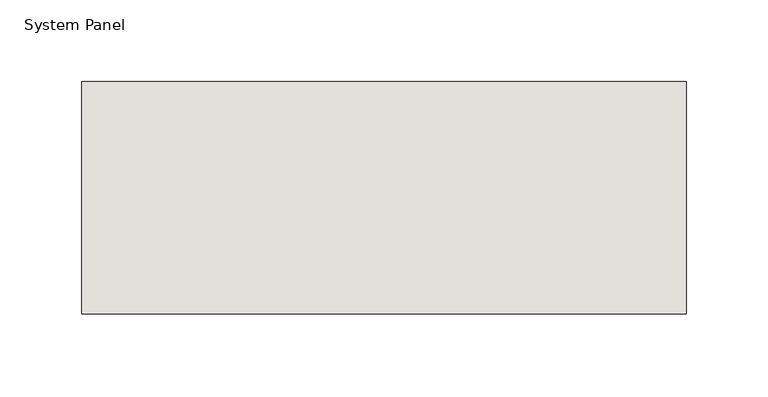
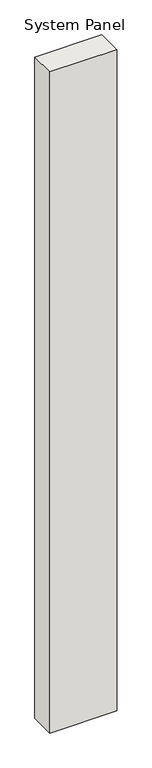
"""IFC4 building model written with IfcOpenShell, lengths in millimetres: wall geometry, System Panel : NLRS_21_CWP_hsb-vulling minerale wol 142 _gen_rsf."""

from ifc_helpers import new_model, si_unit, origin, origin_with_axes, place, context, project, spatial, polyline, outline, extrude, source, transform, mapped, element, save


def system_panel_4b5b3d98(model_context):
    return source(origin(), model_context, "Body", "SweptSolid", [
        extrude(outline(polyline([(184.5, -71.0), (-184.5, -71.0), (-184.5, 71.0), (184.5, 71.0), (184.5, -71.0)])), origin_with_axes(), (0.0, 0.0, 1.0), 3849.0),
    ])


if __name__ == "__main__":
    model = new_model("IFC4")
    model_context = context("Model", 3, world=origin())
    ifc_project = project(units=[si_unit("LENGTHUNIT", "METRE", prefix="MILLI")], contexts=[model_context])
    site = spatial("IfcSite", under=ifc_project)
    building = spatial("IfcBuilding", under=site)
    placement = place(None, origin())
    system_panel_shape = system_panel_4b5b3d98(model_context)
    element("IfcWall", 1, ObjectType="System Panel : NLRS_21_CWP_hsb-vulling minerale wol 142 _gen_rsf", at=placement, inside=building, context=model_context, shape_type="MappedRepresentation", body=[
        mapped(system_panel_shape, transform((0.0, 0.0, 0.0), x_axis=(1.0, 0.0, 0.0), y_axis=(0.0, 1.0, 0.0), z_axis=(0.0, 0.0, 1.0))),
    ])
    save(model, "model.ifc")

# Revit data of these elements
# Type "System Panel : NLRS_21_CWP_hsb-vulling minerale wol 142 _gen_rsf"
#   Type IfcGUID = "07M7mRoiH1CR8m_RSKIwpC"
#   Assembly Code = "21.23"
#   IfcExportAs = "IfcWall"
# Element 1 (IfcWall, "System Panel : NLRS_21_CWP_hsb-vulling minerale wol 142 _gen_rsf")
#   Materials on its faces: "NLRS_m1_isolatie minerale wol_gen_rsf"
# Materials
#   "NLRS_m1_isolatie minerale wol_gen_rsf": class "M - Anorganische materialen", colour RGB 200 200 140, transparency 0, Keynote = "m1", Manufacturer = "Revit Standards Foundation", URL = "www.revitstandards.org", Description = "isolatie minerale wol", Cost = 0
